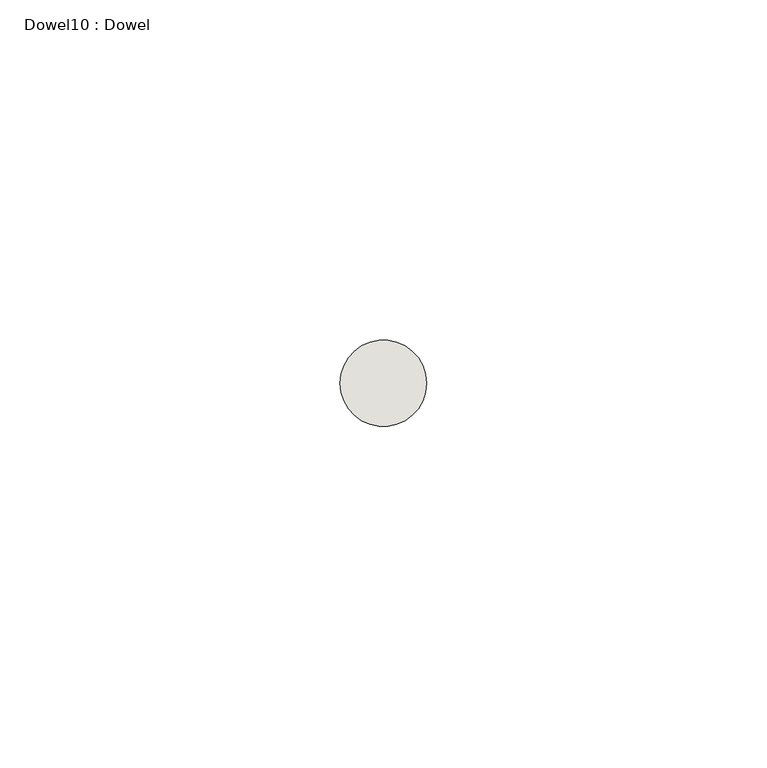
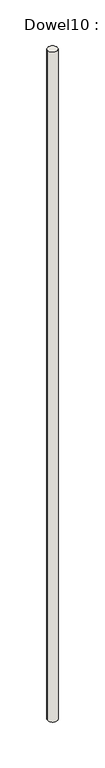
"""IFC4 building model written with IfcOpenShell, lengths in millimetres: wall geometry, Dowel10 : Dowel."""

import ifcopenshell
import ifcopenshell.guid

model = None  # the IFC model being written
_history = None  # IfcOwnerHistory: only IFC2X3 demands one
_inside = {}  # id of a spatial element -> (the spatial element, [elements in it])
_under = {}  # id of a project, library or spatial element -> (it, [spatial elements below it])
_declared = {}  # id of a project -> (the project, [libraries it declares])
_typed = {}  # id of a type object -> (the type object, [elements of that type])
_made_of = {}  # id of a material, layer set ... -> (it, [elements and type objects made of it])


def new_model(schema):
    """Start an empty IFC model of exactly this schema.

    Asked for "IFC4X3", IfcOpenShell would pick the latest addendum, in which some entities
    have other attributes; the version numbers below select the first issue.
    IFC2X3 requires an IfcOwnerHistory on every rooted entity: one is made here for all.
    """
    global model, _history
    if schema == "IFC4X3":
        model = ifcopenshell.file(schema_version=(4, 3, 0, 0))
    else:
        model = ifcopenshell.file(schema=schema)
    _inside.clear()
    _under.clear()
    _declared.clear()
    _typed.clear()
    _made_of.clear()
    _history = None
    if model.schema == "IFC2X3":
        org = make("IfcOrganization", Name="unknown")
        user = make(
            "IfcPersonAndOrganization",
            ThePerson=make("IfcPerson", FamilyName="unknown"),
            TheOrganization=org,
        )
        app = make(
            "IfcApplication",
            ApplicationDeveloper=org,
            Version="unknown",
            ApplicationFullName="unknown",
            ApplicationIdentifier="unknown",
        )
        _history = make(
            "IfcOwnerHistory",
            OwningUser=user,
            OwningApplication=app,
            ChangeAction="ADDED",
            CreationDate=0,
        )
    return model


def make(cls, **values):
    """One entity of the class cls with the attributes given. An attribute that is None is left unset."""
    return model.create_entity(
        cls, **{name: value for name, value in values.items() if value is not None}
    )


def rooted(cls, **values):
    """An entity with a GlobalId (a new one), such as an element, a storey or a relation."""
    return make(cls, GlobalId=ifcopenshell.guid.new(), OwnerHistory=_history, **values)


def si_unit(unit_type, name, prefix=None):
    """IfcSIUnit, for example si_unit("LENGTHUNIT", "METRE", prefix="MILLI")."""
    return make("IfcSIUnit", UnitType=unit_type, Prefix=prefix, Name=name)


def assignment(units):
    """IfcUnitAssignment: the units of a project."""
    return None if units is None else make("IfcUnitAssignment", Units=units)


def point(xyz):
    """IfcCartesianPoint."""
    return None if xyz is None else make("IfcCartesianPoint", Coordinates=xyz)


def direction(xyz):
    """IfcDirection."""
    return None if xyz is None else make("IfcDirection", DirectionRatios=xyz)


def frame(location, z_axis=None, x_axis=None):
    """IfcAxis2Placement3D, a coordinate frame: its origin and axes. An axis left out is left unset."""
    return make(
        "IfcAxis2Placement3D",
        Location=point(location),
        Axis=direction(z_axis),
        RefDirection=direction(x_axis),
    )


def frame_2d(location, x_axis=None):
    """IfcAxis2Placement2D, a coordinate frame in the plane: its origin and x axis."""
    return make(
        "IfcAxis2Placement2D", Location=point(location), RefDirection=direction(x_axis)
    )


def origin():
    """The frame at (0, 0, 0) with its axes left unset."""
    return frame((0.0, 0.0, 0.0))


def place(relative_to, where):
    """IfcLocalPlacement: puts the frame where relative to a parent placement (None: the world)."""
    return make(
        "IfcLocalPlacement", PlacementRelTo=relative_to, RelativePlacement=where
    )


def context(
    kind, dimensions, precision=None, world=None, true_north=None, identifier=None
):
    """IfcGeometricRepresentationContext, for example the 3D "Model" context."""
    return make(
        "IfcGeometricRepresentationContext",
        ContextIdentifier=identifier,
        ContextType=kind,
        CoordinateSpaceDimension=dimensions,
        Precision=precision,
        WorldCoordinateSystem=world,
        TrueNorth=true_north,
    )


def project(units=None, contexts=None):
    """IfcProject with its units and contexts."""
    return rooted(
        "IfcProject",
        Name="project",
        RepresentationContexts=contexts,
        UnitsInContext=assignment(units),
    )


def spatial(cls, under=None, at=None, **own):
    """A site, building, storey or space (cls), placed at a placement, below another one or the project."""
    s = rooted(cls, ObjectPlacement=at, **own)
    if under is not None:
        _under.setdefault(under.id(), (under, []))[1].append(s)
    return s


def circle_curve(where, radius):
    """IfcCircle in the frame where."""
    return make("IfcCircle", Position=where, Radius=radius)


def trimmed(basis, trim1, trim2, sense, master):
    """IfcTrimmedCurve: the piece of a basis curve between two trims."""
    return make(
        "IfcTrimmedCurve",
        BasisCurve=basis,
        Trim1=trim1,
        Trim2=trim2,
        SenseAgreement=sense,
        MasterRepresentation=master,
    )


def segment(curve, same_sense, transition):
    """IfcCompositeCurveSegment."""
    return make(
        "IfcCompositeCurveSegment",
        Transition=transition,
        SameSense=same_sense,
        ParentCurve=curve,
    )


def composite_curve(segments, self_intersect=None):
    """IfcCompositeCurve: segments joined end to end."""
    return make("IfcCompositeCurve", Segments=segments, SelfIntersect=self_intersect)


def outline(outer, holes=None, kind="AREA"):
    """IfcArbitraryClosedProfileDef: a profile drawn as a closed curve; with holes, ...WithVoids."""
    if holes is None:
        return make("IfcArbitraryClosedProfileDef", ProfileType=kind, OuterCurve=outer)
    return make(
        "IfcArbitraryProfileDefWithVoids",
        ProfileType=kind,
        OuterCurve=outer,
        InnerCurves=holes,
    )


def extrude(swept, where, along, depth):
    """IfcExtrudedAreaSolid: the profile swept, set in the frame where, extruded along a direction by depth."""
    return make(
        "IfcExtrudedAreaSolid",
        SweptArea=swept,
        Position=where,
        ExtrudedDirection=direction(along),
        Depth=depth,
    )


def shape(context_of_items, identifier, shape_type, items):
    """IfcShapeRepresentation: the items that make up one representation, for example the "Body"."""
    return make(
        "IfcShapeRepresentation",
        ContextOfItems=context_of_items,
        RepresentationIdentifier=identifier,
        RepresentationType=shape_type,
        Items=items,
    )


def source(mapping_origin, context_of_items, identifier, shape_type, items):
    """IfcRepresentationMap: a shape defined once, which mapped items show again and again."""
    return make(
        "IfcRepresentationMap",
        MappingOrigin=mapping_origin,
        MappedRepresentation=shape(context_of_items, identifier, shape_type, items),
    )


def transform(
    local_origin,
    x_axis=None,
    y_axis=None,
    z_axis=None,
    scale=None,
    scale2=None,
    scale3=None,
    uniform=True,
):
    """IfcCartesianTransformationOperator3D, or its non-uniform kind. x_axis, y_axis, z_axis: its Axis1, 2, 3."""
    if uniform:
        return make(
            "IfcCartesianTransformationOperator3D",
            Axis1=direction(x_axis),
            Axis2=direction(y_axis),
            LocalOrigin=point(local_origin),
            Scale=scale,
            Axis3=direction(z_axis),
        )
    return make(
        "IfcCartesianTransformationOperator3DnonUniform",
        Axis1=direction(x_axis),
        Axis2=direction(y_axis),
        LocalOrigin=point(local_origin),
        Scale=scale,
        Axis3=direction(z_axis),
        Scale2=scale2,
        Scale3=scale3,
    )


def mapped(mapping_source, mapping_target):
    """IfcMappedItem: shows the shape of a source again, moved by a transform."""
    return make(
        "IfcMappedItem", MappingSource=mapping_source, MappingTarget=mapping_target
    )


def made_of(thing, what):
    """Note that an element or type object is made of a material, layer set ...; save() writes the relation."""
    if what is not None:
        _made_of.setdefault(what.id(), (what, []))[1].append(thing)
    return thing


def element(
    cls,
    number,
    at=None,
    inside=None,
    cuts=None,
    type_object=None,
    material=None,
    context=None,
    identifier="Body",
    shape_type=None,
    held_by="IfcProductDefinitionShape",
    body=None,
    shapes=None,
    **own,
):
    """One element of the class cls, such as IfcWall. Its Tag is "e" and its number.

    at: its placement. inside: the storey or other place that contains it. cuts: it is an
    opening in that element (IfcRelVoidsElement). A single representation is given by context,
    identifier, shape_type and body (its items); several are given by shapes. held_by: the class
    of the entity that holds the representations. save() writes the other relations.
    """
    e = rooted(cls, Tag="e%d" % number, ObjectPlacement=at, **own)
    if body is not None:
        shapes = [shape(context, identifier, shape_type, body)]
    if shapes is not None:
        e.Representation = make(held_by, Representations=shapes)
    if inside is not None:
        _inside.setdefault(inside.id(), (inside, []))[1].append(e)
    if cuts is not None:
        rooted(
            "IfcRelVoidsElement", RelatingBuildingElement=cuts, RelatedOpeningElement=e
        )
    if type_object is not None:
        _typed.setdefault(type_object.id(), (type_object, []))[1].append(e)
    return made_of(e, material)


def aggregate(whole, parts):
    """IfcRelAggregates: a whole, such as a stair, and the parts it consists of."""
    return rooted("IfcRelAggregates", RelatingObject=whole, RelatedObjects=parts)


def save(model, path):
    """Write the relations noted so far, then the file.

    IfcRelAggregates (storeys below a building ...), IfcRelContainedInSpatialStructure (elements
    in a storey), IfcRelDefinesByType, IfcRelAssociatesMaterial and IfcRelDeclares: one each for
    every whole, place, type object, material and project.
    """
    for whole, parts in _under.values():
        aggregate(whole, parts)
    for where, things in _inside.values():
        rooted(
            "IfcRelContainedInSpatialStructure",
            RelatedElements=things,
            RelatingStructure=where,
        )
    for kind, things in _typed.values():
        rooted("IfcRelDefinesByType", RelatedObjects=things, RelatingType=kind)
    for what, things in _made_of.values():
        rooted("IfcRelAssociatesMaterial", RelatedObjects=things, RelatingMaterial=what)
    for by, libraries in _declared.values():
        rooted("IfcRelDeclares", RelatingContext=by, RelatedDefinitions=libraries)
    model.write(path)


def dowel10_dowel_0302f649(model_context):
    return source(origin(), model_context, "Body", "SweptSolid", [
        extrude(outline(composite_curve([segment(trimmed(circle_curve(frame_2d((376532.7748047, 446.88125)), 6.35), [point((376526.4248047, 446.88125))], [point((376539.1248047, 446.88125))], False, "CARTESIAN"), True, "CONTINUOUS"), segment(trimmed(circle_curve(frame_2d((376532.7748047, 446.88125)), 6.35), [point((376539.1248047, 446.88125))], [point((376526.4248047, 446.88125))], False, "CARTESIAN"), True, "CONTINUOUS")], self_intersect=False)), frame((0.0, 0.0, 1679.6089342), z_axis=(0.0, 0.0, 1.0), x_axis=(1.0, 0.0, 0.0)), (0.0, 0.0, 1.0), 914.4),
    ])


if __name__ == "__main__":
    model = new_model("IFC4")
    model_context = context("Model", 3, world=origin())
    ifc_project = project(units=[si_unit("LENGTHUNIT", "METRE", prefix="MILLI")], contexts=[model_context])
    site = spatial("IfcSite", under=ifc_project)
    building = spatial("IfcBuilding", under=site)
    placement = place(None, origin())
    dowel10_dowel_shape = dowel10_dowel_0302f649(model_context)
    element("IfcWall", 1, ObjectType="Dowel10 : Dowel", at=placement, inside=building, context=model_context, shape_type="MappedRepresentation", body=[
        mapped(dowel10_dowel_shape, transform((0.0, 0.0, 0.0), x_axis=(1.0, 0.0, 0.0), y_axis=(0.0, 1.0, 0.0), z_axis=(0.0, 0.0, 1.0))),
    ])
    save(model, "model.ifc")

# Revit data of these elements
# Element 1 (IfcWall, "Dowel10 : Dowel")
#   Materials on its faces: "#4 VERTICAL U-SHAPED HAIRPINS AT 18\" O.C. - 36\" LONG"
# Materials
#   "#4 VERTICAL U-SHAPED HAIRPINS AT 18\" O.C. - 36\" LONG": class "Generic", colour RGB 255 255 255, transparency 0, Cost = 0
